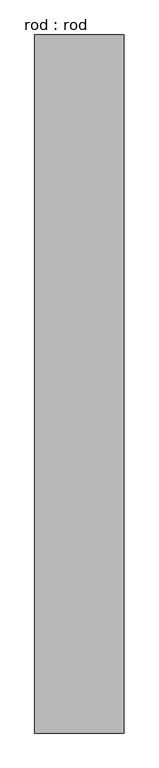
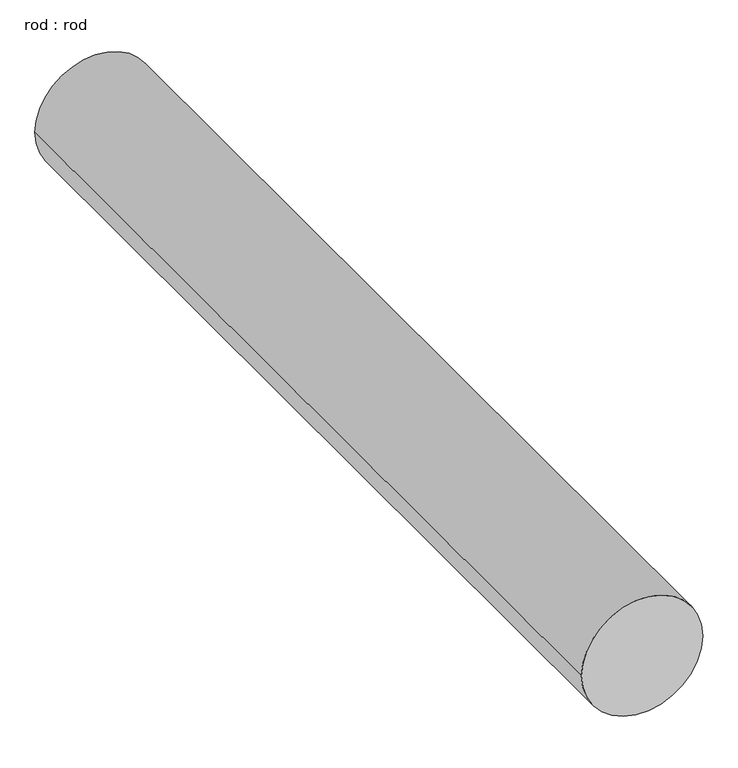
"""IFC4 building model written with IfcOpenShell, lengths in millimetres: proxy geometry, rod : rod."""

from ifc_helpers import new_model, si_unit, point, frame, frame_2d, origin, place, context, project, spatial, circle_curve, trimmed, segment, composite_curve, outline, extrude, source, transform, mapped, element, save


def rod_rod_9d8cd088(model_context):
    return source(origin(), model_context, "Body", "SweptSolid", [
        extrude(outline(composite_curve([segment(trimmed(circle_curve(frame_2d((0.0108462, 0.0)), 200.0), [point((0.0108462, 200.0))], [point((0.0108462, -200.0))], False, "CARTESIAN"), True, "CONTINUOUS"), segment(trimmed(circle_curve(frame_2d((0.0108462, 0.0)), 200.0), [point((0.0108462, -200.0))], [point((0.0108462, 200.0))], False, "CARTESIAN"), True, "CONTINUOUS")], self_intersect=False)), frame((0.0, 2528.4429011, 0.0), z_axis=(0.0, 1.0, 0.0), x_axis=(0.0, 0.0, 1.0)), (0.0, 0.0, 1.0), 3128.5714286),
    ])


if __name__ == "__main__":
    model = new_model("IFC4")
    model_context = context("Model", 3, world=origin())
    ifc_project = project(units=[si_unit("LENGTHUNIT", "METRE", prefix="MILLI")], contexts=[model_context])
    site = spatial("IfcSite", under=ifc_project)
    building = spatial("IfcBuilding", under=site)
    placement = place(None, origin())
    rod_rod_shape = rod_rod_9d8cd088(model_context)
    element("IfcBuildingElementProxy", 1, Name="rod : rod", ObjectType="rod : rod", at=placement, inside=building, context=model_context, shape_type="MappedRepresentation", body=[
        mapped(rod_rod_shape, transform((0.0, 0.0, 0.0), x_axis=(1.0, 0.0, 0.0), y_axis=(0.0, 1.0, 0.0), z_axis=(0.0, 0.0, 1.0))),
    ])
    save(model, "model.ifc")

# Revit data of these elements
# Type "rod : rod"
#   Default Elevation = 0
